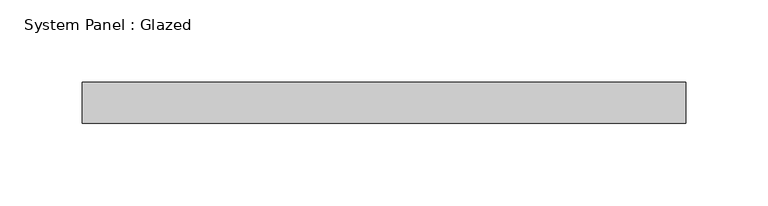
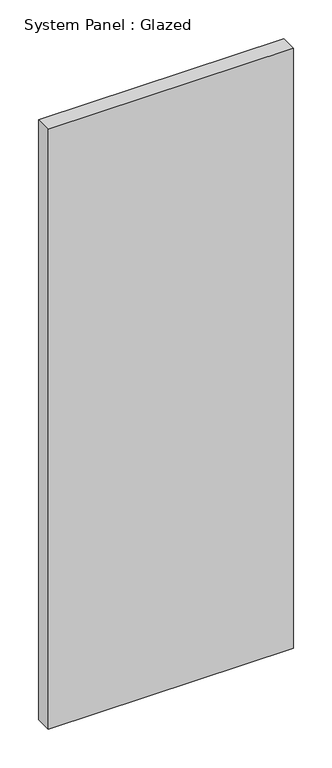
"""IFC4 building model written with IfcOpenShell, lengths in millimetres: plate geometry, System Panel : Glazed."""

from ifc_helpers import new_model, si_unit, origin, origin_with_axes, place, context, project, spatial, polyline, outline, extrude, source, transform, mapped, element, save


def system_panel_glazed_3ec057d3(model_context):
    return source(origin(), model_context, "Body", "SweptSolid", [
        extrude(outline(polyline([(183.8383838, 24.5), (-183.8383838, 24.5), (-183.8383838, 49.5), (183.8383838, 49.5), (183.8383838, 24.5)])), origin_with_axes(), (0.0, 0.0, 1.0), 950.0),
    ])


if __name__ == "__main__":
    model = new_model("IFC4")
    model_context = context("Model", 3, world=origin())
    ifc_project = project(units=[si_unit("LENGTHUNIT", "METRE", prefix="MILLI")], contexts=[model_context])
    site = spatial("IfcSite", under=ifc_project)
    building = spatial("IfcBuilding", under=site)
    placement = place(None, origin())
    system_panel_glazed_shape = system_panel_glazed_3ec057d3(model_context)
    element("IfcPlate", 1, ObjectType="System Panel : Glazed", at=placement, inside=building, context=model_context, shape_type="MappedRepresentation", body=[
        mapped(system_panel_glazed_shape, transform((0.0, 0.0, 0.0), x_axis=(1.0, 0.0, 0.0), y_axis=(0.0, 1.0, 0.0), z_axis=(0.0, 0.0, 1.0))),
    ])
    save(model, "model.ifc")

# Revit data of these elements
# Element 1 (IfcPlate, "System Panel : Glazed")
#   Materials on its faces: "Glass"
# Materials
#   "Glass": class "Glass", colour RGB 218 227 224, transparency 0.85, Description = "Soda Lime Glass", Cost = 0
